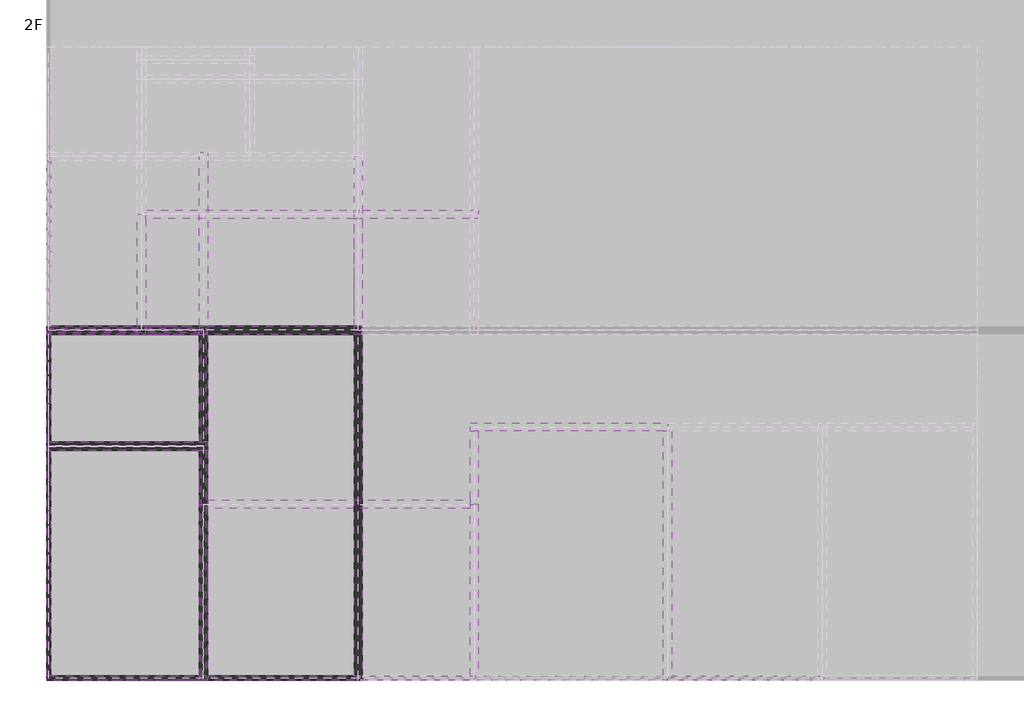
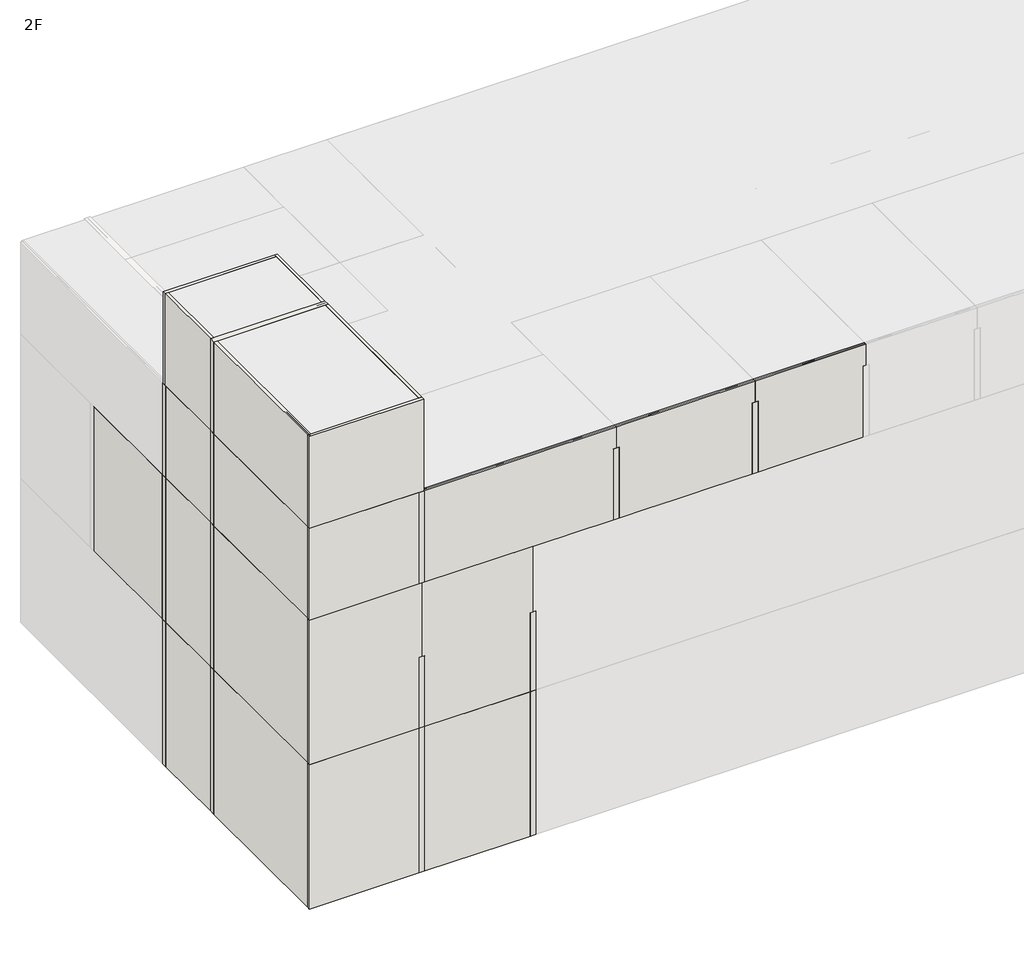
# One storey, part 1 of 3: 51 walls.
"""IFC4 building model written with IfcOpenShell, lengths in millimetres."""

from ifc_helpers import new_model, si_unit, frame, origin, place, context, project, spatial, polyline, outline, extrude, faceted_brep, element, save

model = new_model("IFC4")

# Units and contexts
model_context = context("Model", 3, world=origin())
ifc_project = project(units=[si_unit("LENGTHUNIT", "METRE", prefix="MILLI")], contexts=[model_context])

# Site, building, storey
site = spatial("IfcSite", under=ifc_project)
building = spatial("IfcBuilding", under=site)
storey = spatial("IfcBuildingStorey", under=building, Name="2F", Elevation=3500.0)

# Walls
placement = place(None, origin())
element("IfcWall", 1, ObjectType="WA211_Exterior-Cement Brick-90mm", at=placement, inside=storey, context=model_context, shape_type="SweptSolid", body=[
    extrude(outline(polyline([(49566.6521483, 163980.8614395), (53352.6521483, 163980.8614395), (53352.6521483, 163866.8614395), (49566.6521483, 163866.8614395), (49566.6521483, 163980.8614395)])), frame((0.0, 0.0, 3500.0), z_axis=(0.0, 0.0, 1.0), x_axis=(1.0, 0.0, 0.0)), (0.0, 0.0, 1.0), 5500.0),
])
element("IfcWall", 2, ObjectType="WA211_Exterior-Cement Brick-90mm", at=placement, inside=storey, context=model_context, shape_type="SweptSolid", body=[
    extrude(outline(polyline([(45516.6521483, 172816.8614395), (45516.6521483, 170030.8614395), (45402.6521483, 170030.8614395), (45402.6521483, 172816.8614395), (45516.6521483, 172816.8614395)])), frame((0.0, 0.0, 3500.0), z_axis=(0.0, 0.0, 1.0), x_axis=(1.0, 0.0, 0.0)), (0.0, 0.0, 1.0), 5500.0),
])
element("IfcWall", 3, ObjectType="WA211_Exterior-Cement Brick-90mm", at=placement, inside=storey, context=model_context, shape_type="SweptSolid", body=[
    extrude(outline(polyline([(45516.6521483, 169816.8614395), (45516.6521483, 163980.8614395), (45402.6521483, 163980.8614395), (45402.6521483, 169816.8614395), (45516.6521483, 169816.8614395)])), frame((0.0, 0.0, 3500.0), z_axis=(0.0, 0.0, 1.0), x_axis=(1.0, 0.0, 0.0)), (0.0, 0.0, 1.0), 5500.0),
])
element("IfcWall", 4, ObjectType="WA211_Exterior-Cement Brick-90mm", at=placement, inside=storey, context=model_context, shape_type="Brep", body=[
    faceted_brep([(49352.6521483, 163980.8614395, 3500.0), (45516.6521483, 163980.8614395, 3500.0), (45402.6521483, 163980.8614395, 3500.0), (45402.6521483, 163980.8614395, 9000.0), (45516.6521483, 163980.8614395, 9000.0), (49352.6521483, 163980.8614395, 9000.0), (49352.6521483, 163866.8614395, 3500.0), (49352.6521483, 163866.8614395, 9000.0), (45402.6521483, 163866.8614395, 9000.0), (45402.6521483, 163866.8614395, 3500.0)], [[[0, 1, 2, 3, 4, 5]], [[6, 7, 8, 9]], [[2, 1, 0, 6, 9]], [[5, 4, 3, 8, 7]], [[0, 5, 7, 6]], [[3, 2, 9, 8]]]),
])
element("IfcWall", 5, ObjectType="WA211_Exterior-Cement Brick-90mm", at=placement, inside=storey, context=model_context, shape_type="SweptSolid", body=[
    extrude(outline(polyline([(45516.6521483, 177316.8614395), (45516.6521483, 173030.8614395), (45402.6521483, 173030.8614395), (45402.6521483, 177316.8614395), (45516.6521483, 177316.8614395)])), frame((0.0, 0.0, 9000.0), z_axis=(0.0, 0.0, 1.0), x_axis=(1.0, 0.0, 0.0)), (0.0, 0.0, 1.0), 5500.0),
])
element("IfcWall", 6, ObjectType="WA211_Exterior-Cement Brick-90mm", at=placement, inside=storey, context=model_context, shape_type="SweptSolid", body=[
    extrude(outline(polyline([(45516.6521483, 172816.8614395), (45516.6521483, 170030.8614395), (45402.6521483, 170030.8614395), (45402.6521483, 172816.8614395), (45516.6521483, 172816.8614395)])), frame((0.0, 0.0, 9000.0), z_axis=(0.0, 0.0, 1.0), x_axis=(1.0, 0.0, 0.0)), (0.0, 0.0, 1.0), 5500.0),
])
element("IfcWall", 7, ObjectType="WA211_Exterior-Cement Brick-90mm", at=placement, inside=storey, context=model_context, shape_type="SweptSolid", body=[
    extrude(outline(polyline([(45516.6521483, 169816.8614395), (45516.6521483, 163980.8614395), (45402.6521483, 163980.8614395), (45402.6521483, 169816.8614395), (45516.6521483, 169816.8614395)])), frame((0.0, 0.0, 9000.0), z_axis=(0.0, 0.0, 1.0), x_axis=(1.0, 0.0, 0.0)), (0.0, 0.0, 1.0), 5500.0),
])
element("IfcWall", 8, ObjectType="WA211_Exterior-Cement Brick-90mm", at=placement, inside=storey, context=model_context, shape_type="Brep", body=[
    faceted_brep([(49352.6521483, 163980.8614395, 9000.0), (45516.6521483, 163980.8614395, 9000.0), (45402.6521483, 163980.8614395, 9000.0), (45402.6521483, 163980.8614395, 14500.0), (45516.6521483, 163980.8614395, 14500.0), (49459.6521483, 163980.8614395, 14500.0), (49459.6521483, 163980.8614395, 11700.0), (49352.6521483, 163980.8614395, 11700.0), (49352.6521483, 163866.8614395, 9000.0), (49352.6521483, 163866.8614395, 11700.0), (49459.6521483, 163866.8614395, 11700.0), (49459.6521483, 163866.8614395, 14500.0), (45402.6521483, 163866.8614395, 14500.0), (45402.6521483, 163866.8614395, 9000.0)], [[[0, 1, 2, 3, 4, 5, 6, 7]], [[8, 9, 10, 11, 12, 13]], [[2, 1, 0, 8, 13]], [[5, 4, 3, 12, 11]], [[3, 2, 13, 12]], [[6, 5, 11, 10]], [[6, 10, 9, 7]], [[0, 7, 9, 8]]]),
])
element("IfcWall", 9, ObjectType="WA211_Exterior-Cement Brick-90mm", at=placement, inside=storey, context=model_context, shape_type="SweptSolid", body=[
    extrude(outline(polyline([(9000.0, 53352.6521483), (12000.0, 53352.6521483), (12000.0, 53459.6521483), (14500.0, 53459.6521483), (14500.0, 49459.6521483), (11700.0, 49459.6521483), (11700.0, 49566.6521483), (9000.0, 49566.6521483), (9000.0, 53352.6521483)])), frame((0.0, 163866.8614395, 0.0), z_axis=(0.0, 1.0, 0.0), x_axis=(0.0, 0.0, 1.0)), (0.0, 0.0, 1.0), 114.0),
])
element("IfcWall", 10, ObjectType="WA211_Exterior-Cement Brick-90mm", at=placement, inside=storey, context=model_context, shape_type="SweptSolid", body=[
    extrude(outline(polyline([(14500.0, 65352.6521483), (17200.0, 65352.6521483), (17200.0, 65459.6521483), (18000.0, 65459.6521483), (18000.0, 61459.6521483), (17200.0, 61459.6521483), (17200.0, 61566.6521483), (14500.0, 61566.6521483), (14500.0, 65352.6521483)])), frame((0.0, 163866.8614395, 0.0), z_axis=(0.0, 1.0, 0.0), x_axis=(0.0, 0.0, 1.0)), (0.0, 0.0, 1.0), 114.0),
])
element("IfcWall", 11, ObjectType="WA211_Exterior-Cement Brick-90mm", at=placement, inside=storey, context=model_context, shape_type="SweptSolid", body=[
    extrude(outline(polyline([(14500.0, 61352.6521483), (17200.0, 61352.6521483), (17200.0, 61459.6521483), (18000.0, 61459.6521483), (18000.0, 56459.6521483), (17200.0, 56459.6521483), (17200.0, 56566.6521483), (14500.0, 56566.6521483), (14500.0, 61352.6521483)])), frame((0.0, 163866.8614395, 0.0), z_axis=(0.0, 1.0, 0.0), x_axis=(0.0, 0.0, 1.0)), (0.0, 0.0, 1.0), 114.0),
])
element("IfcWall", 12, ObjectType="WA211_Exterior-Cement Brick-90mm", at=placement, inside=storey, context=model_context, shape_type="SweptSolid", body=[
    extrude(outline(polyline([(14500.0, 56352.6521483), (17200.0, 56352.6521483), (17200.0, 56459.6521483), (18000.0, 56459.6521483), (18000.0, 49566.6521483), (14500.0, 49566.6521483), (14500.0, 56352.6521483)])), frame((0.0, 163866.8614395, 0.0), z_axis=(0.0, 1.0, 0.0), x_axis=(0.0, 0.0, 1.0)), (0.0, 0.0, 1.0), 114.0),
])
element("IfcWall", 13, ObjectType="WA211_Exterior-Cement Brick-90mm", at=placement, inside=storey, context=model_context, shape_type="SweptSolid", body=[
    extrude(outline(polyline([(45516.6521483, 172816.8614395), (45516.6521483, 170030.8614395), (45402.6521483, 170030.8614395), (45402.6521483, 172816.8614395), (45516.6521483, 172816.8614395)])), frame((0.0, 0.0, 14500.0), z_axis=(0.0, 0.0, 1.0), x_axis=(1.0, 0.0, 0.0)), (0.0, 0.0, 1.0), 3500.0),
])
element("IfcWall", 14, ObjectType="WA211_Exterior-Cement Brick-90mm", at=placement, inside=storey, context=model_context, shape_type="SweptSolid", body=[
    extrude(outline(polyline([(45516.6521483, 169816.8614395), (45516.6521483, 163980.8614395), (45402.6521483, 163980.8614395), (45402.6521483, 169816.8614395), (45516.6521483, 169816.8614395)])), frame((0.0, 0.0, 14500.0), z_axis=(0.0, 0.0, 1.0), x_axis=(1.0, 0.0, 0.0)), (0.0, 0.0, 1.0), 3500.0),
])
element("IfcWall", 15, ObjectType="WA211_Exterior-Cement Brick-90mm", at=placement, inside=storey, context=model_context, shape_type="Brep", body=[
    faceted_brep([(49352.6521483, 163980.8614395, 14500.0), (45516.6521483, 163980.8614395, 14500.0), (45402.6521483, 163980.8614395, 14500.0), (45402.6521483, 163980.8614395, 18000.0), (45516.6521483, 163980.8614395, 18000.0), (49352.6521483, 163980.8614395, 18000.0), (49352.6521483, 163866.8614395, 14500.0), (49352.6521483, 163866.8614395, 18000.0), (45402.6521483, 163866.8614395, 18000.0), (45402.6521483, 163866.8614395, 14500.0)], [[[0, 1, 2, 3, 4, 5]], [[6, 7, 8, 9]], [[2, 1, 0, 6, 9]], [[5, 4, 3, 8, 7]], [[0, 5, 7, 6]], [[3, 2, 9, 8]]]),
])
element("IfcWall", 16, ObjectType="WA211_Exterior-Cement Brick-90mm", at=placement, inside=storey, context=model_context, shape_type="Brep", body=[
    faceted_brep([(49402.6521483, 172980.8614395, 18000.0), (49402.6521483, 172866.8614395, 18000.0), (49402.6521483, 170030.8614395, 18000.0), (49402.6521483, 170030.8614395, 21500.0), (49402.6521483, 172866.8614395, 21500.0), (49402.6521483, 172980.8614395, 21500.0), (49516.6521483, 172980.8614395, 18000.0), (49516.6521483, 172980.8614395, 21500.0), (49516.6521483, 170030.8614395, 21500.0), (49516.6521483, 170030.8614395, 18000.0)], [[[0, 1, 2, 3, 4, 5]], [[6, 7, 8, 9]], [[2, 1, 0, 6, 9]], [[5, 4, 3, 8, 7]], [[0, 5, 7, 6]], [[3, 2, 9, 8]]]),
])
element("IfcWall", 17, ObjectType="WA211_Exterior-Cement Brick-90mm", at=placement, inside=storey, context=model_context, shape_type="SweptSolid", body=[
    extrude(outline(polyline([(45516.6521483, 172866.8614395), (45516.6521483, 170030.8614395), (45402.6521483, 170030.8614395), (45402.6521483, 172866.8614395), (45516.6521483, 172866.8614395)])), frame((0.0, 0.0, 18000.0), z_axis=(0.0, 0.0, 1.0), x_axis=(1.0, 0.0, 0.0)), (0.0, 0.0, 1.0), 3500.0),
])
element("IfcWall", 18, ObjectType="WA211_Exterior-Cement Brick-90mm", at=placement, inside=storey, context=model_context, shape_type="Brep", body=[
    faceted_brep([(45402.6521483, 172866.8614395, 18000.0), (45516.6521483, 172866.8614395, 18000.0), (49402.6521483, 172866.8614395, 18000.0), (49402.6521483, 172866.8614395, 21500.0), (45516.6521483, 172866.8614395, 21500.0), (45402.6521483, 172866.8614395, 21500.0), (45402.6521483, 172980.8614395, 18000.0), (45402.6521483, 172980.8614395, 21500.0), (49402.6521483, 172980.8614395, 21500.0), (49402.6521483, 172980.8614395, 18000.0)], [[[0, 1, 2, 3, 4, 5]], [[6, 7, 8, 9]], [[2, 1, 0, 6, 9]], [[5, 4, 3, 8, 7]], [[0, 5, 7, 6]], [[3, 2, 9, 8]]]),
])
element("IfcWall", 19, ObjectType="WA211_Exterior-Cement Brick-90mm", at=placement, inside=storey, context=model_context, shape_type="SweptSolid", body=[
    extrude(outline(polyline([(45516.6521483, 169816.8614395), (45516.6521483, 163980.8614395), (45402.6521483, 163980.8614395), (45402.6521483, 169816.8614395), (45516.6521483, 169816.8614395)])), frame((0.0, 0.0, 18000.0), z_axis=(0.0, 0.0, 1.0), x_axis=(1.0, 0.0, 0.0)), (0.0, 0.0, 1.0), 3500.0),
])
element("IfcWall", 20, ObjectType="WA211_Exterior-Cement Brick-90mm", at=placement, inside=storey, context=model_context, shape_type="Brep", body=[
    faceted_brep([(49516.6521483, 163980.8614395, 18000.0), (49402.6521483, 163980.8614395, 18000.0), (45516.6521483, 163980.8614395, 18000.0), (45402.6521483, 163980.8614395, 18000.0), (45402.6521483, 163980.8614395, 21500.0), (45516.6521483, 163980.8614395, 21500.0), (49402.6521483, 163980.8614395, 21500.0), (49516.6521483, 163980.8614395, 21500.0), (49516.6521483, 163866.8614395, 18000.0), (49516.6521483, 163866.8614395, 21500.0), (45402.6521483, 163866.8614395, 21500.0), (45402.6521483, 163866.8614395, 18000.0)], [[[0, 1, 2, 3, 4, 5, 6, 7]], [[8, 9, 10, 11]], [[3, 2, 1, 0, 8, 11]], [[7, 6, 5, 4, 10, 9]], [[0, 7, 9, 8]], [[4, 3, 11, 10]]]),
])
element("IfcWall", 21, ObjectType="WA211_Exterior-Cement Brick-90mm", at=placement, inside=storey, context=model_context, shape_type="SweptSolid", body=[
    extrude(outline(polyline([(49402.6521483, 163980.8614395), (49402.6521483, 169816.8614395), (49516.6521483, 169816.8614395), (49516.6521483, 163980.8614395), (49402.6521483, 163980.8614395)])), frame((0.0, 0.0, 18000.0), z_axis=(0.0, 0.0, 1.0), x_axis=(1.0, 0.0, 0.0)), (0.0, 0.0, 1.0), 3500.0),
])
element("IfcWall", 22, ObjectType="WA221_Interior-Cement Block-190mm", at=placement, inside=storey, context=model_context, shape_type="SweptSolid", body=[
    extrude(outline(polyline([(49566.6521483, 173030.8614395), (53352.6521483, 173030.8614395), (53352.6521483, 172816.8614395), (49566.6521483, 172816.8614395), (49566.6521483, 173030.8614395)])), frame((0.0, 0.0, 3500.0), z_axis=(0.0, 0.0, 1.0), x_axis=(1.0, 0.0, 0.0)), (0.0, 0.0, 1.0), 5500.0),
])
element("IfcWall", 23, ObjectType="WA221_Interior-Cement Block-190mm", at=placement, inside=storey, context=model_context, shape_type="Brep", body=[
    faceted_brep([(45402.6521483, 172816.8614395, 3500.0), (45516.6521483, 172816.8614395, 3500.0), (49352.6521483, 172816.8614395, 3500.0), (49352.6521483, 172816.8614395, 9000.0), (45516.6521483, 172816.8614395, 9000.0), (45402.6521483, 172816.8614395, 9000.0), (45402.6521483, 173030.8614395, 3500.0), (45402.6521483, 173030.8614395, 9000.0), (45516.6521483, 173030.8614395, 9000.0), (49352.6521483, 173030.8614395, 9000.0), (49352.6521483, 173030.8614395, 3500.0), (45516.6521483, 173030.8614395, 3500.0)], [[[0, 1, 2, 3, 4, 5]], [[6, 7, 8, 9, 10, 11]], [[2, 1, 0, 6, 11, 10]], [[5, 4, 3, 9, 8, 7]], [[0, 5, 7, 6]], [[3, 2, 10, 9]]]),
])
element("IfcWall", 24, ObjectType="WA221_Interior-Cement Block-190mm", at=placement, inside=storey, context=model_context, shape_type="Brep", body=[
    faceted_brep([(53566.6521483, 163866.8614395, 3500.0), (53566.6521483, 163980.8614395, 3500.0), (53566.6521483, 172816.8614395, 3500.0), (53566.6521483, 173030.8614395, 3500.0), (53566.6521483, 173030.8614395, 9000.0), (53566.6521483, 172816.8614395, 9000.0), (53566.6521483, 163980.8614395, 9000.0), (53566.6521483, 163866.8614395, 9000.0), (53352.6521483, 163866.8614395, 3500.0), (53352.6521483, 163866.8614395, 9000.0), (53352.6521483, 163980.8614395, 9000.0), (53352.6521483, 172816.8614395, 9000.0), (53352.6521483, 173030.8614395, 9000.0), (53352.6521483, 173030.8614395, 3500.0), (53352.6521483, 172816.8614395, 3500.0), (53352.6521483, 163980.8614395, 3500.0)], [[[0, 1, 2, 3, 4, 5, 6, 7]], [[8, 9, 10, 11, 12, 13, 14, 15]], [[3, 2, 1, 0, 8, 15, 14, 13]], [[7, 6, 5, 4, 12, 11, 10, 9]], [[0, 7, 9, 8]], [[4, 3, 13, 12]]]),
])
element("IfcWall", 25, ObjectType="WA221_Interior-Cement Block-190mm", at=placement, inside=storey, context=model_context, shape_type="Brep", body=[
    faceted_brep([(49352.6521483, 173030.8614395, 3500.0), (49352.6521483, 172816.8614395, 3500.0), (49352.6521483, 170030.8614395, 3500.0), (49352.6521483, 170030.8614395, 9000.0), (49352.6521483, 172816.8614395, 9000.0), (49352.6521483, 173030.8614395, 9000.0), (49566.6521483, 173030.8614395, 3500.0), (49566.6521483, 173030.8614395, 9000.0), (49566.6521483, 172816.8614395, 9000.0), (49566.6521483, 170030.8614395, 9000.0), (49566.6521483, 170030.8614395, 3500.0), (49566.6521483, 172816.8614395, 3500.0)], [[[0, 1, 2, 3, 4, 5]], [[6, 7, 8, 9, 10, 11]], [[2, 1, 0, 6, 11, 10]], [[5, 4, 3, 9, 8, 7]], [[0, 5, 7, 6]], [[3, 2, 10, 9]]]),
])
element("IfcWall", 26, ObjectType="WA221_Interior-Cement Block-190mm", at=placement, inside=storey, context=model_context, shape_type="Brep", body=[
    faceted_brep([(49352.6521483, 169816.8614395, 3500.0), (49352.6521483, 163980.8614395, 3500.0), (49352.6521483, 163866.8614395, 3500.0), (49352.6521483, 163866.8614395, 9000.0), (49352.6521483, 163980.8614395, 9000.0), (49352.6521483, 169816.8614395, 9000.0), (49566.6521483, 169816.8614395, 3500.0), (49566.6521483, 169816.8614395, 9000.0), (49566.6521483, 163980.8614395, 9000.0), (49566.6521483, 163866.8614395, 9000.0), (49566.6521483, 163866.8614395, 3500.0), (49566.6521483, 163980.8614395, 3500.0)], [[[0, 1, 2, 3, 4, 5]], [[6, 7, 8, 9, 10, 11]], [[2, 1, 0, 6, 11, 10]], [[5, 4, 3, 9, 8, 7]], [[3, 2, 10, 9]], [[0, 5, 7, 6]]]),
])
element("IfcWall", 27, ObjectType="WA221_Interior-Cement Block-190mm", at=placement, inside=storey, context=model_context, shape_type="Brep", body=[
    faceted_brep([(45402.6521483, 169816.8614395, 3500.0), (45516.6521483, 169816.8614395, 3500.0), (49352.6521483, 169816.8614395, 3500.0), (49566.6521483, 169816.8614395, 3500.0), (49566.6521483, 169816.8614395, 9000.0), (49352.6521483, 169816.8614395, 9000.0), (45516.6521483, 169816.8614395, 9000.0), (45402.6521483, 169816.8614395, 9000.0), (45402.6521483, 170030.8614395, 3500.0), (45402.6521483, 170030.8614395, 9000.0), (45516.6521483, 170030.8614395, 9000.0), (49352.6521483, 170030.8614395, 9000.0), (49566.6521483, 170030.8614395, 9000.0), (49566.6521483, 170030.8614395, 3500.0), (49352.6521483, 170030.8614395, 3500.0), (45516.6521483, 170030.8614395, 3500.0)], [[[0, 1, 2, 3, 4, 5, 6, 7]], [[8, 9, 10, 11, 12, 13, 14, 15]], [[3, 2, 1, 0, 8, 15, 14, 13]], [[7, 6, 5, 4, 12, 11, 10, 9]], [[0, 7, 9, 8]], [[4, 3, 13, 12]]]),
])
element("IfcWall", 28, ObjectType="WA221_Interior-Cement Block-190mm", at=placement, inside=storey, context=model_context, shape_type="Brep", body=[
    faceted_brep([(53566.6521483, 172923.8614395, 9000.0), (53566.6521483, 173030.8614395, 9000.0), (53566.6521483, 177316.8614395, 9000.0), (53566.6521483, 177316.8614395, 11700.0), (53566.6521483, 177423.8614395, 11700.0), (53566.6521483, 177423.8614395, 12400.0), (53566.6521483, 173030.8614395, 12400.0), (53566.6521483, 172816.8614395, 12400.0), (53566.6521483, 172816.8614395, 12000.0), (53566.6521483, 172923.8614395, 12000.0), (53352.6521483, 172923.8614395, 9000.0), (53352.6521483, 172923.8614395, 12000.0), (53352.6521483, 172816.8614395, 12000.0), (53352.6521483, 172816.8614395, 12400.0), (53352.6521483, 177423.8614395, 12400.0), (53352.6521483, 177423.8614395, 11700.0), (53352.6521483, 177316.8614395, 11700.0), (53352.6521483, 177316.8614395, 9000.0)], [[[0, 1, 2, 3, 4, 5, 6, 7, 8, 9]], [[10, 11, 12, 13, 14, 15, 16, 17]], [[2, 1, 0, 10, 17]], [[7, 6, 5, 14, 13]], [[0, 9, 11, 10]], [[8, 12, 11, 9]], [[8, 7, 13, 12]], [[5, 4, 15, 14]], [[15, 4, 3, 16]], [[3, 2, 17, 16]]]),
])
element("IfcWall", 29, ObjectType="WA221_Interior-Cement Block-190mm", at=placement, inside=storey, context=model_context, shape_type="Brep", body=[
    faceted_brep([(53566.6521483, 163866.8614395, 9000.0), (53566.6521483, 163980.8614395, 9000.0), (53566.6521483, 172816.8614395, 9000.0), (53566.6521483, 172923.8614395, 9000.0), (53566.6521483, 172923.8614395, 12000.0), (53566.6521483, 172816.8614395, 12000.0), (53566.6521483, 163980.8614395, 12000.0), (53566.6521483, 163866.8614395, 12000.0), (53352.6521483, 163866.8614395, 9000.0), (53352.6521483, 163866.8614395, 12000.0), (53352.6521483, 163980.8614395, 12000.0), (53352.6521483, 172816.8614395, 12000.0), (53352.6521483, 172923.8614395, 12000.0), (53352.6521483, 172923.8614395, 9000.0), (53352.6521483, 163980.8614395, 9000.0), (53459.6521483, 163866.8614395, 12000.0)], [[[0, 1, 2, 3, 4, 5, 6, 7]], [[8, 9, 10, 11, 12, 13, 14]], [[3, 2, 1, 0, 8, 14, 13]], [[4, 3, 13, 12]], [[7, 6, 5, 4, 12, 11, 10, 9, 15]], [[0, 7, 15, 9, 8]]]),
])
element("IfcWall", 30, ObjectType="WA221_Interior-Cement Block-190mm", at=placement, inside=storey, context=model_context, shape_type="Brep", body=[
    faceted_brep([(45402.6521483, 172816.8614395, 9000.0), (45516.6521483, 172816.8614395, 9000.0), (49352.6521483, 172816.8614395, 9000.0), (49566.6521483, 172816.8614395, 9000.0), (49566.6521483, 172816.8614395, 14500.0), (49352.6521483, 172816.8614395, 14500.0), (45516.6521483, 172816.8614395, 14500.0), (45402.6521483, 172816.8614395, 14500.0), (45402.6521483, 173030.8614395, 9000.0), (45402.6521483, 173030.8614395, 14500.0), (45516.6521483, 173030.8614395, 14500.0), (49566.6521483, 173030.8614395, 14500.0), (49566.6521483, 173030.8614395, 11700.0), (49566.6521483, 173030.8614395, 9000.0), (49352.6521483, 173030.8614395, 9000.0), (45516.6521483, 173030.8614395, 9000.0)], [[[0, 1, 2, 3, 4, 5, 6, 7]], [[8, 9, 10, 11, 12, 13, 14, 15]], [[3, 2, 1, 0, 8, 15, 14, 13]], [[7, 6, 5, 4, 11, 10, 9]], [[0, 7, 9, 8]], [[3, 13, 12, 11, 4]]]),
])
element("IfcWall", 31, ObjectType="WA221_Interior-Cement Block-190mm", at=placement, inside=storey, context=model_context, shape_type="Brep", body=[
    faceted_brep([(49352.6521483, 177530.8614395, 9000.0), (49352.6521483, 177316.8614395, 9000.0), (49352.6521483, 173030.8614395, 9000.0), (49352.6521483, 173030.8614395, 11700.0), (49352.6521483, 177316.8614395, 11700.0), (49352.6521483, 177530.8614395, 11700.0), (49566.6521483, 177530.8614395, 9000.0), (49566.6521483, 177530.8614395, 11700.0), (49566.6521483, 177316.8614395, 11700.0), (49566.6521483, 173030.8614395, 11700.0), (49566.6521483, 173030.8614395, 9000.0), (49566.6521483, 177316.8614395, 9000.0)], [[[0, 1, 2, 3, 4, 5]], [[6, 7, 8, 9, 10, 11]], [[2, 1, 0, 6, 11, 10]], [[5, 4, 3, 9, 8, 7]], [[0, 5, 7, 6]], [[3, 2, 10, 9]]]),
])
element("IfcWall", 32, ObjectType="WA221_Interior-Cement Block-190mm", at=placement, inside=storey, context=model_context, shape_type="Brep", body=[
    faceted_brep([(49566.6521483, 170030.8614395, 14500.0), (49566.6521483, 170030.8614395, 9000.0), (49352.6521483, 170030.8614395, 9000.0), (45516.6521483, 170030.8614395, 9000.0), (45402.6521483, 170030.8614395, 9000.0), (45402.6521483, 170030.8614395, 14500.0), (45516.6521483, 170030.8614395, 14500.0), (49352.6521483, 170030.8614395, 14500.0), (49566.6521483, 169816.8614395, 9000.0), (49566.6521483, 169816.8614395, 11700.0), (49566.6521483, 169816.8614395, 14500.0), (45516.6521483, 169816.8614395, 14500.0), (45402.6521483, 169816.8614395, 14500.0), (45402.6521483, 169816.8614395, 9000.0), (45516.6521483, 169816.8614395, 9000.0), (49352.6521483, 169816.8614395, 9000.0)], [[[0, 1, 2, 3, 4, 5, 6, 7]], [[8, 9, 10, 11, 12, 13, 14, 15]], [[4, 3, 2, 1, 8, 15, 14, 13]], [[0, 7, 6, 5, 12, 11, 10]], [[5, 4, 13, 12]], [[0, 10, 9, 8, 1]]]),
])
element("IfcWall", 33, ObjectType="WA221_Interior-Cement Block-190mm", at=placement, inside=storey, context=model_context, shape_type="SweptSolid", body=[
    extrude(outline(polyline([(49352.6521483, 170030.8614395), (49352.6521483, 172816.8614395), (49566.6521483, 172816.8614395), (49566.6521483, 170030.8614395), (49352.6521483, 170030.8614395)])), frame((0.0, 0.0, 9000.0), z_axis=(0.0, 0.0, 1.0), x_axis=(1.0, 0.0, 0.0)), (0.0, 0.0, 1.0), 5500.0),
])
element("IfcWall", 34, ObjectType="WA221_Interior-Cement Block-190mm", at=placement, inside=storey, context=model_context, shape_type="Brep", body=[
    faceted_brep([(49352.6521483, 169816.8614395, 9000.0), (49352.6521483, 163980.8614395, 9000.0), (49352.6521483, 163866.8614395, 9000.0), (49352.6521483, 163866.8614395, 11700.0), (49352.6521483, 163980.8614395, 11700.0), (49352.6521483, 169816.8614395, 11700.0), (49566.6521483, 169816.8614395, 9000.0), (49566.6521483, 169816.8614395, 11700.0), (49566.6521483, 163980.8614395, 11700.0), (49566.6521483, 163866.8614395, 11700.0), (49566.6521483, 163866.8614395, 9000.0), (49566.6521483, 163980.8614395, 9000.0), (49459.6521483, 163866.8614395, 11700.0)], [[[0, 1, 2, 3, 4, 5]], [[6, 7, 8, 9, 10, 11]], [[2, 1, 0, 6, 11, 10]], [[5, 4, 3, 12, 9, 8, 7]], [[0, 5, 7, 6]], [[3, 2, 10, 9, 12]]]),
])
element("IfcWall", 35, ObjectType="WA221_Interior-Cement Block-190mm", at=placement, inside=storey, context=model_context, shape_type="Brep", body=[
    faceted_brep([(61352.6521483, 170316.8614395, 14500.0), (61352.6521483, 163980.8614395, 14500.0), (61352.6521483, 163866.8614395, 14500.0), (61352.6521483, 163866.8614395, 17200.0), (61352.6521483, 163980.8614395, 17200.0), (61352.6521483, 170316.8614395, 17200.0), (61566.6521483, 170316.8614395, 14500.0), (61566.6521483, 170316.8614395, 17200.0), (61566.6521483, 163980.8614395, 17200.0), (61566.6521483, 163866.8614395, 17200.0), (61566.6521483, 163866.8614395, 14500.0), (61566.6521483, 163980.8614395, 14500.0), (61459.6521483, 170316.8614395, 14500.0), (61459.6521483, 163866.8614395, 17200.0), (61459.6521483, 170316.8614395, 17200.0)], [[[0, 1, 2, 3, 4, 5]], [[6, 7, 8, 9, 10, 11]], [[2, 1, 0, 12, 6, 11, 10]], [[5, 4, 3, 13, 9, 8, 7, 14]], [[3, 2, 10, 9, 13]], [[0, 5, 14, 7, 6, 12]]]),
])
element("IfcWall", 36, ObjectType="WA221_Interior-Cement Block-190mm", at=placement, inside=storey, context=model_context, shape_type="Brep", body=[
    faceted_brep([(56566.6521483, 163866.8614395, 14500.0), (56566.6521483, 163980.8614395, 14500.0), (56566.6521483, 168423.8614395, 14500.0), (56566.6521483, 168423.8614395, 17200.0), (56566.6521483, 163980.8614395, 17200.0), (56566.6521483, 163866.8614395, 17200.0), (56352.6521483, 163866.8614395, 14500.0), (56352.6521483, 163866.8614395, 17200.0), (56352.6521483, 163980.8614395, 17200.0), (56352.6521483, 168316.8614395, 17200.0), (56352.6521483, 168423.8614395, 17200.0), (56352.6521483, 168423.8614395, 14500.0), (56352.6521483, 168316.8614395, 14500.0), (56352.6521483, 163980.8614395, 14500.0), (56459.6521483, 163866.8614395, 17200.0)], [[[0, 1, 2, 3, 4, 5]], [[6, 7, 8, 9, 10, 11, 12, 13]], [[2, 1, 0, 6, 13, 12, 11]], [[3, 2, 11, 10]], [[5, 4, 3, 10, 9, 8, 7, 14]], [[0, 5, 14, 7, 6]]]),
])
element("IfcWall", 37, ObjectType="WA221_Interior-Cement Block-190mm", at=placement, inside=storey, context=model_context, shape_type="Brep", body=[
    faceted_brep([(56352.6521483, 170316.8614395, 14500.0), (56566.6521483, 170316.8614395, 14500.0), (61352.6521483, 170316.8614395, 14500.0), (61459.6521483, 170316.8614395, 14500.0), (61459.6521483, 170316.8614395, 17200.0), (61352.6521483, 170316.8614395, 17200.0), (56566.6521483, 170316.8614395, 17200.0), (56352.6521483, 170316.8614395, 17200.0), (56352.6521483, 170530.8614395, 14500.0), (56352.6521483, 170530.8614395, 17200.0), (61459.6521483, 170530.8614395, 17200.0), (61459.6521483, 170530.8614395, 14500.0)], [[[0, 1, 2, 3, 4, 5, 6, 7]], [[8, 9, 10, 11]], [[3, 2, 1, 0, 8, 11]], [[4, 3, 11, 10]], [[7, 6, 5, 4, 10, 9]], [[0, 7, 9, 8]]]),
])
element("IfcWall", 38, ObjectType="WA221_Interior-Cement Block-190mm", at=placement, inside=storey, context=model_context, shape_type="Brep", body=[
    faceted_brep([(56566.6521483, 168423.8614395, 14500.0), (56566.6521483, 170316.8614395, 14500.0), (56566.6521483, 170316.8614395, 17200.0), (56566.6521483, 168423.8614395, 17200.0), (56352.6521483, 168423.8614395, 14500.0), (56352.6521483, 168423.8614395, 17200.0), (56352.6521483, 168530.8614395, 17200.0), (56352.6521483, 170316.8614395, 17200.0), (56352.6521483, 170316.8614395, 14500.0), (56352.6521483, 168530.8614395, 14500.0)], [[[0, 1, 2, 3]], [[4, 5, 6, 7, 8, 9]], [[1, 0, 4, 9, 8]], [[3, 2, 7, 6, 5]], [[0, 3, 5, 4]], [[2, 1, 8, 7]]]),
])
element("IfcWall", 39, ObjectType="WA221_Interior-Cement Block-190mm", at=placement, inside=storey, context=model_context, shape_type="Brep", body=[
    faceted_brep([(49352.6521483, 168423.8614395, 18000.0), (49352.6521483, 168423.8614395, 14500.0), (49352.6521483, 163980.8614395, 14500.0), (49352.6521483, 163866.8614395, 14500.0), (49352.6521483, 163866.8614395, 18000.0), (49352.6521483, 163980.8614395, 18000.0), (49566.6521483, 168423.8614395, 14500.0), (49566.6521483, 168423.8614395, 18000.0), (49566.6521483, 163980.8614395, 18000.0), (49566.6521483, 163866.8614395, 18000.0), (49566.6521483, 163866.8614395, 14500.0), (49566.6521483, 163980.8614395, 14500.0), (49566.6521483, 168316.8614395, 14500.0)], [[[0, 1, 2, 3, 4, 5]], [[6, 7, 8, 9, 10, 11, 12]], [[3, 2, 1, 6, 12, 11, 10]], [[0, 5, 4, 9, 8, 7]], [[0, 7, 6, 1]], [[4, 3, 10, 9]]]),
])
element("IfcWall", 40, ObjectType="WA221_Interior-Cement Block-190mm", at=placement, inside=storey, context=model_context, shape_type="Brep", body=[
    faceted_brep([(56352.6521483, 168530.8614395, 14500.0), (49566.6521483, 168530.8614395, 14500.0), (49566.6521483, 168530.8614395, 17200.0), (56352.6521483, 168530.8614395, 17200.0), (56352.6521483, 168316.8614395, 14500.0), (56352.6521483, 168316.8614395, 17200.0), (49566.6521483, 168316.8614395, 17200.0), (49566.6521483, 168316.8614395, 14500.0), (56352.6521483, 168423.8614395, 14500.0), (49566.6521483, 168423.8614395, 14500.0), (56352.6521483, 168423.8614395, 17200.0)], [[[0, 1, 2, 3]], [[4, 5, 6, 7]], [[1, 0, 8, 4, 7, 9]], [[3, 2, 6, 5, 10]], [[0, 3, 10, 5, 4, 8]], [[2, 1, 9, 7, 6]]]),
])
element("IfcWall", 41, ObjectType="WA221_Interior-Cement Block-190mm", at=placement, inside=storey, context=model_context, shape_type="Brep", body=[
    faceted_brep([(47966.6521483, 175816.8614395, 14500.0), (53352.6521483, 175816.8614395, 14500.0), (53459.6521483, 175816.8614395, 14500.0), (53459.6521483, 175816.8614395, 17200.0), (53352.6521483, 175816.8614395, 17200.0), (47966.6521483, 175816.8614395, 17200.0), (47966.6521483, 176030.8614395, 14500.0), (47966.6521483, 176030.8614395, 17200.0), (53352.6521483, 176030.8614395, 17200.0), (53459.6521483, 176030.8614395, 17200.0), (53459.6521483, 176030.8614395, 14500.0), (53352.6521483, 176030.8614395, 14500.0), (47966.6521483, 175923.8614395, 14500.0)], [[[0, 1, 2, 3, 4, 5]], [[6, 7, 8, 9, 10, 11]], [[2, 1, 0, 12, 6, 11, 10]], [[3, 2, 10, 9]], [[5, 4, 3, 9, 8, 7]], [[0, 5, 7, 6, 12]]]),
])
element("IfcWall", 42, ObjectType="WA221_Interior-Cement Block-190mm", at=placement, inside=storey, context=model_context, shape_type="Brep", body=[
    faceted_brep([(53459.6521483, 175816.8614395, 14500.0), (53566.6521483, 175816.8614395, 14500.0), (56352.6521483, 175816.8614395, 14500.0), (56566.6521483, 175816.8614395, 14500.0), (56566.6521483, 175816.8614395, 17200.0), (56352.6521483, 175816.8614395, 17200.0), (53566.6521483, 175816.8614395, 17200.0), (53459.6521483, 175816.8614395, 17200.0), (53459.6521483, 176030.8614395, 14500.0), (53459.6521483, 176030.8614395, 17200.0), (53566.6521483, 176030.8614395, 17200.0), (56352.6521483, 176030.8614395, 17200.0), (56566.6521483, 176030.8614395, 17200.0), (56566.6521483, 176030.8614395, 14500.0), (56352.6521483, 176030.8614395, 14500.0), (53566.6521483, 176030.8614395, 14500.0)], [[[0, 1, 2, 3, 4, 5, 6, 7]], [[8, 9, 10, 11, 12, 13, 14, 15]], [[3, 2, 1, 0, 8, 15, 14, 13]], [[7, 6, 5, 4, 12, 11, 10, 9]], [[0, 7, 9, 8]], [[4, 3, 13, 12]]]),
])
element("IfcWall", 43, ObjectType="WA221_Interior-Cement Block-190mm", at=placement, inside=storey, context=model_context, shape_type="Brep", body=[
    faceted_brep([(47752.6521483, 175923.8614395, 18000.0), (47752.6521483, 175923.8614395, 14500.0), (47752.6521483, 173030.8614395, 14500.0), (47752.6521483, 172816.8614395, 14500.0), (47752.6521483, 172816.8614395, 18000.0), (47752.6521483, 173030.8614395, 18000.0), (47966.6521483, 175923.8614395, 14500.0), (47966.6521483, 175923.8614395, 18000.0), (47966.6521483, 173030.8614395, 18000.0), (47966.6521483, 172816.8614395, 18000.0), (47966.6521483, 172816.8614395, 14500.0), (47966.6521483, 173030.8614395, 14500.0), (47966.6521483, 175816.8614395, 14500.0)], [[[0, 1, 2, 3, 4, 5]], [[6, 7, 8, 9, 10, 11, 12]], [[3, 2, 1, 6, 12, 11, 10]], [[0, 5, 4, 9, 8, 7]], [[0, 7, 6, 1]], [[4, 3, 10, 9]]]),
])
element("IfcWall", 44, ObjectType="WA221_Interior-Cement Block-190mm", at=placement, inside=storey, context=model_context, shape_type="SweptSolid", body=[
    extrude(outline(polyline([(49352.6521483, 172816.8614395), (47966.6521483, 172816.8614395), (47966.6521483, 173030.8614395), (49352.6521483, 173030.8614395), (49352.6521483, 172816.8614395)])), frame((0.0, 0.0, 14500.0), z_axis=(0.0, 0.0, 1.0), x_axis=(1.0, 0.0, 0.0)), (0.0, 0.0, 1.0), 3500.0),
])
element("IfcWall", 45, ObjectType="WA221_Interior-Cement Block-190mm", at=placement, inside=storey, context=model_context, shape_type="Brep", body=[
    faceted_brep([(53566.6521483, 173030.8614395, 14500.0), (53352.6521483, 173030.8614395, 14500.0), (49566.6521483, 173030.8614395, 14500.0), (49566.6521483, 173030.8614395, 17200.0), (53352.6521483, 173030.8614395, 17200.0), (53566.6521483, 173030.8614395, 17200.0), (53566.6521483, 172816.8614395, 14500.0), (53566.6521483, 172816.8614395, 17200.0), (49566.6521483, 172816.8614395, 17200.0), (49566.6521483, 172816.8614395, 14500.0)], [[[0, 1, 2, 3, 4, 5]], [[6, 7, 8, 9]], [[2, 1, 0, 6, 9]], [[5, 4, 3, 8, 7]], [[0, 5, 7, 6]], [[3, 2, 9, 8]]]),
])
element("IfcWall", 46, ObjectType="WA221_Interior-Cement Block-190mm", at=placement, inside=storey, context=model_context, shape_type="Brep", body=[
    faceted_brep([(53352.6521483, 175816.8614395, 14500.0), (53352.6521483, 173030.8614395, 14500.0), (53352.6521483, 173030.8614395, 17200.0), (53352.6521483, 175816.8614395, 17200.0), (53566.6521483, 175816.8614395, 14500.0), (53566.6521483, 175816.8614395, 17200.0), (53566.6521483, 173030.8614395, 17200.0), (53566.6521483, 173030.8614395, 14500.0), (53459.6521483, 175816.8614395, 14500.0), (53459.6521483, 175816.8614395, 17200.0)], [[[0, 1, 2, 3]], [[4, 5, 6, 7]], [[1, 0, 8, 4, 7]], [[3, 2, 6, 5, 9]], [[0, 3, 9, 5, 4, 8]], [[2, 1, 7, 6]]]),
])
element("IfcWall", 47, ObjectType="WA221_Interior-Cement Block-190mm", at=placement, inside=storey, context=model_context, shape_type="Brep", body=[
    faceted_brep([(47752.6521483, 173030.8614395, 14500.0), (45516.6521483, 173030.8614395, 14500.0), (45402.6521483, 173030.8614395, 14500.0), (45402.6521483, 173030.8614395, 18000.0), (45516.6521483, 173030.8614395, 18000.0), (47752.6521483, 173030.8614395, 18000.0), (47752.6521483, 172816.8614395, 14500.0), (47752.6521483, 172816.8614395, 18000.0), (45516.6521483, 172816.8614395, 18000.0), (45402.6521483, 172816.8614395, 18000.0), (45402.6521483, 172816.8614395, 14500.0), (45516.6521483, 172816.8614395, 14500.0)], [[[0, 1, 2, 3, 4, 5]], [[6, 7, 8, 9, 10, 11]], [[2, 1, 0, 6, 11, 10]], [[5, 4, 3, 9, 8, 7]], [[0, 5, 7, 6]], [[3, 2, 10, 9]]]),
])
element("IfcWall", 48, ObjectType="WA221_Interior-Cement Block-190mm", at=placement, inside=storey, context=model_context, shape_type="Brep", body=[
    faceted_brep([(45402.6521483, 169816.8614395, 14500.0), (45516.6521483, 169816.8614395, 14500.0), (49352.6521483, 169816.8614395, 14500.0), (49566.6521483, 169816.8614395, 14500.0), (49566.6521483, 169816.8614395, 18000.0), (49352.6521483, 169816.8614395, 18000.0), (45516.6521483, 169816.8614395, 18000.0), (45402.6521483, 169816.8614395, 18000.0), (45402.6521483, 170030.8614395, 14500.0), (45402.6521483, 170030.8614395, 18000.0), (45516.6521483, 170030.8614395, 18000.0), (49352.6521483, 170030.8614395, 18000.0), (49566.6521483, 170030.8614395, 18000.0), (49566.6521483, 170030.8614395, 14500.0), (49352.6521483, 170030.8614395, 14500.0), (45516.6521483, 170030.8614395, 14500.0)], [[[0, 1, 2, 3, 4, 5, 6, 7]], [[8, 9, 10, 11, 12, 13, 14, 15]], [[3, 2, 1, 0, 8, 15, 14, 13]], [[7, 6, 5, 4, 12, 11, 10, 9]], [[0, 7, 9, 8]], [[4, 3, 13, 12]]]),
])
element("IfcWall", 49, ObjectType="WA221_Interior-Cement Block-190mm", at=placement, inside=storey, context=model_context, shape_type="Brep", body=[
    faceted_brep([(49352.6521483, 173030.8614395, 18000.0), (49352.6521483, 173030.8614395, 14500.0), (49352.6521483, 172816.8614395, 14500.0), (49352.6521483, 170030.8614395, 14500.0), (49352.6521483, 170030.8614395, 18000.0), (49352.6521483, 172816.8614395, 18000.0), (49566.6521483, 173030.8614395, 14500.0), (49566.6521483, 173030.8614395, 17200.0), (49566.6521483, 173030.8614395, 18000.0), (49566.6521483, 170030.8614395, 18000.0), (49566.6521483, 170030.8614395, 14500.0), (49566.6521483, 172816.8614395, 14500.0)], [[[0, 1, 2, 3, 4, 5]], [[6, 7, 8, 9, 10, 11]], [[3, 2, 1, 6, 11, 10]], [[0, 5, 4, 9, 8]], [[4, 3, 10, 9]], [[0, 8, 7, 6, 1]]]),
])
element("IfcWall", 50, ObjectType="WA221_Interior-Cement Block-190mm", at=placement, inside=storey, context=model_context, shape_type="Brep", body=[
    faceted_brep([(49352.6521483, 169816.8614395, 14500.0), (49352.6521483, 168423.8614395, 14500.0), (49352.6521483, 168423.8614395, 18000.0), (49352.6521483, 169816.8614395, 18000.0), (49566.6521483, 169816.8614395, 14500.0), (49566.6521483, 169816.8614395, 18000.0), (49566.6521483, 168423.8614395, 18000.0), (49566.6521483, 168423.8614395, 14500.0), (49566.6521483, 168530.8614395, 14500.0)], [[[0, 1, 2, 3]], [[4, 5, 6, 7, 8]], [[1, 0, 4, 8, 7]], [[3, 2, 6, 5]], [[1, 7, 6, 2]], [[0, 3, 5, 4]]]),
])
element("IfcWall", 51, ObjectType="WA221_Interior-Cement Block-190mm", at=placement, inside=storey, context=model_context, shape_type="Brep", body=[
    faceted_brep([(49516.6521483, 170030.8614395, 18000.0), (49402.6521483, 170030.8614395, 18000.0), (45516.6521483, 170030.8614395, 18000.0), (45402.6521483, 170030.8614395, 18000.0), (45402.6521483, 170030.8614395, 21500.0), (45516.6521483, 170030.8614395, 21500.0), (49402.6521483, 170030.8614395, 21500.0), (49516.6521483, 170030.8614395, 21500.0), (49516.6521483, 169816.8614395, 18000.0), (49516.6521483, 169816.8614395, 21500.0), (49402.6521483, 169816.8614395, 21500.0), (45516.6521483, 169816.8614395, 21500.0), (45402.6521483, 169816.8614395, 21500.0), (45402.6521483, 169816.8614395, 18000.0), (45516.6521483, 169816.8614395, 18000.0), (49402.6521483, 169816.8614395, 18000.0)], [[[0, 1, 2, 3, 4, 5, 6, 7]], [[8, 9, 10, 11, 12, 13, 14, 15]], [[3, 2, 1, 0, 8, 15, 14, 13]], [[7, 6, 5, 4, 12, 11, 10, 9]], [[0, 7, 9, 8]], [[4, 3, 13, 12]]]),
])

save(model, "model.ifc")

# Revit data of these elements
# Type "WA211_Exterior-Cement Brick-90mm"
#   Type Comments = ""
#   Layers, outside or top first: 0 mm "A04AL081-00001_Skirt_Acrylic Emulsion Paint" (function 100); 0 mm "A04AL077-00001_Ext Wall Painting_Acrylic Emulsion Paint" (function 100); 12 mm "A04AS164-00001_Plastering_Ext" (function 4); 90 mm "A04AK073-00001_Concrete Brick_0.5B" (function 1); 12 mm "A04AS164-00002_Plastering_Int" (function 5); 0 mm "A04AL078-00002_Int Wall Painting_Water Emulsion Paint" (function 100); 0 mm "A04AL081-00001_Skirt_Acrylic Emulsion Paint" (function 100)
# Type "WA221_Interior-Cement Block-190mm"
#   Type Comments = ""
#   Layers, outside or top first: 0 mm "A04AL081-00001_Skirt_Acrylic Emulsion Paint" (function 100); 0 mm "A04AL078-00002_Int Wall Painting_Water Emulsion Paint" (function 100); 12 mm "A04AS164-00002_Plastering_Int" (function 2); 190 mm "A04AK069-00002_Reinforced Concrete Block_THK 100-200mm" (function 1); 12 mm "A04AS164-00002_Plastering_Int" (function 2); 0 mm "A04AL078-00002_Int Wall Painting_Water Emulsion Paint" (function 100); 0 mm "A04AL081-00001_Skirt_Acrylic Emulsion Paint" (function 100)
# Elements 1, 2, 3 (IfcWall, "WA211_Exterior-Cement Brick-90mm")
#   Top Offset = 0 mm
#   Base Offset = 0 mm
#   Unconnected Height = 5500 mm
#   wall height = 5500 mm
#   Phase Created = New Construction
#   Base Constraint = 2F
#   Materials on its faces: "Default Wall", "A04AS164-00002_Plastering_Int", "A04AS164-00001_Plastering_Ext"
# Element 4 (IfcWall, "WA211_Exterior-Cement Brick-90mm")
#   Top Offset = 0 mm
#   Base Offset = 0 mm
#   Unconnected Height = 5500 mm
#   wall height = 5500 mm
#   Phase Created = New Construction
#   Base Constraint = 2F
#   Materials on its faces: "Default Wall", "A04AS164-00001_Plastering_Ext", "A04AS164-00002_Plastering_Int"
# Elements 5, 6, 7, 9 (IfcWall, "WA211_Exterior-Cement Brick-90mm")
#   Top Offset = 0 mm
#   Base Offset = 0 mm
#   Unconnected Height = 5500 mm
#   wall height = 5500 mm
#   Phase Created = New Construction
#   Base Constraint = 3F
#   Materials on its faces: "Default Wall", "A04AS164-00002_Plastering_Int", "A04AS164-00001_Plastering_Ext"
# Element 8 (IfcWall, "WA211_Exterior-Cement Brick-90mm")
#   Top Offset = 0 mm
#   Base Offset = 0 mm
#   Unconnected Height = 5500 mm
#   wall height = 5500 mm
#   Phase Created = New Construction
#   Base Constraint = 3F
#   Materials on its faces: "Default Wall", "A04AS164-00001_Plastering_Ext", "A04AS164-00002_Plastering_Int"
# Elements 10, 11, 12, 13, 14 (IfcWall, "WA211_Exterior-Cement Brick-90mm")
#   Top Offset = 0 mm
#   Base Offset = 0 mm
#   Unconnected Height = 3500 mm
#   wall height = 3500 mm
#   Phase Created = New Construction
#   Base Constraint = 4F
#   Materials on its faces: "Default Wall", "A04AS164-00002_Plastering_Int", "A04AS164-00001_Plastering_Ext"
# Element 15 (IfcWall, "WA211_Exterior-Cement Brick-90mm")
#   Top Offset = 0 mm
#   Base Offset = 0 mm
#   Unconnected Height = 3500 mm
#   wall height = 3500 mm
#   Phase Created = New Construction
#   Base Constraint = 4F
#   Materials on its faces: "Default Wall", "A04AS164-00001_Plastering_Ext", "A04AS164-00002_Plastering_Int"
# Elements 16, 18 (IfcWall, "WA211_Exterior-Cement Brick-90mm")
#   Top Offset = 0 mm
#   Base Offset = 0 mm
#   Unconnected Height = 3500 mm
#   wall height = 3500 mm
#   Phase Created = New Construction
#   Base Constraint = PF
#   Materials on its faces: "Default Wall", "A04AS164-00001_Plastering_Ext", "A04AS164-00002_Plastering_Int"
# Elements 17, 19, 21 (IfcWall, "WA211_Exterior-Cement Brick-90mm")
#   Top Offset = 0 mm
#   Base Offset = 0 mm
#   Unconnected Height = 3500 mm
#   wall height = 3500 mm
#   Phase Created = New Construction
#   Base Constraint = PF
#   Materials on its faces: "Default Wall", "A04AS164-00002_Plastering_Int", "A04AS164-00001_Plastering_Ext"
# Element 20 (IfcWall, "WA211_Exterior-Cement Brick-90mm")
#   Top Offset = 0 mm
#   Base Offset = 0 mm
#   Unconnected Height = 3500 mm
#   wall height = 3500 mm
#   Phase Created = New Construction
#   Base Constraint = PF
#   Materials on its faces: "A04AS164-00001_Plastering_Ext", "Default Wall", "A04AS164-00002_Plastering_Int"
# Element 22 (IfcWall, "WA221_Interior-Cement Block-190mm")
#   Top Offset = 0 mm
#   Base Offset = 0 mm
#   Unconnected Height = 5500 mm
#   wall height = 5500 mm
#   Phase Created = New Construction
#   Base Constraint = 2F
#   Materials on its faces: "Default Wall", "A04AS164-00002_Plastering_Int"
# Elements 23, 26 (IfcWall, "WA221_Interior-Cement Block-190mm")
#   Top Offset = 0 mm
#   Base Offset = 0 mm
#   Unconnected Height = 5500 mm
#   wall height = 5500 mm
#   Phase Created = New Construction
#   Base Constraint = 2F
#   Materials on its faces: "Default Wall", "A04AS164-00002_Plastering_Int", "A04AS164-00001_Plastering_Ext"
# Elements 24, 27 (IfcWall, "WA221_Interior-Cement Block-190mm")
#   Top Offset = 0 mm
#   Base Offset = 0 mm
#   Unconnected Height = 5500 mm
#   wall height = 5500 mm
#   Phase Created = New Construction
#   Base Constraint = 2F
#   Materials on its faces: "A04AS164-00002_Plastering_Int", "Default Wall", "A04AS164-00001_Plastering_Ext"
# Element 25 (IfcWall, "WA221_Interior-Cement Block-190mm")
#   Top Offset = 0 mm
#   Base Offset = 0 mm
#   Unconnected Height = 5500 mm
#   wall height = 5500 mm
#   Phase Created = New Construction
#   Base Constraint = 2F
#   Materials on its faces: "A04AS164-00002_Plastering_Int", "Default Wall"
# Element 28 (IfcWall, "WA221_Interior-Cement Block-190mm")
#   Top Offset = 0 mm
#   Base Offset = 0 mm
#   Unconnected Height = 3400 mm
#   wall height = 3400 mm
#   Phase Created = New Construction
#   Base Constraint = 3F
#   Materials on its faces: "Default Wall", "A04AS164-00002_Plastering_Int"
# Element 29 (IfcWall, "WA221_Interior-Cement Block-190mm")
#   Top Offset = 0 mm
#   Base Offset = 0 mm
#   Unconnected Height = 3000 mm
#   wall height = 3000 mm
#   Phase Created = New Construction
#   Base Constraint = 3F
#   Materials on its faces: "Default Wall", "A04AS164-00002_Plastering_Int", "A04AS164-00001_Plastering_Ext"
# Elements 30, 32 (IfcWall, "WA221_Interior-Cement Block-190mm")
#   Top Offset = 0 mm
#   Base Offset = 0 mm
#   Unconnected Height = 5500 mm
#   wall height = 5500 mm
#   Phase Created = New Construction
#   Base Constraint = 3F
#   Materials on its faces: "A04AS164-00002_Plastering_Int", "Default Wall", "A04AS164-00001_Plastering_Ext"
# Element 31 (IfcWall, "WA221_Interior-Cement Block-190mm")
#   Top Offset = 0 mm
#   Base Offset = 0 mm
#   Unconnected Height = 2700 mm
#   wall height = 2700 mm
#   Phase Created = New Construction
#   Base Constraint = 3F
#   Materials on its faces: "A04AS164-00002_Plastering_Int", "Default Wall"
# Element 33 (IfcWall, "WA221_Interior-Cement Block-190mm")
#   Top Offset = 0 mm
#   Base Offset = 0 mm
#   Unconnected Height = 5500 mm
#   wall height = 5500 mm
#   Phase Created = New Construction
#   Base Constraint = 3F
#   Materials on its faces: "Default Wall", "A04AS164-00002_Plastering_Int"
# Element 34 (IfcWall, "WA221_Interior-Cement Block-190mm")
#   Top Offset = 0 mm
#   Base Offset = 0 mm
#   Unconnected Height = 2700 mm
#   wall height = 2700 mm
#   Phase Created = New Construction
#   Base Constraint = 3F
#   Materials on its faces: "Default Wall", "A04AS164-00002_Plastering_Int", "A04AS164-00001_Plastering_Ext"
# Elements 35, 36 (IfcWall, "WA221_Interior-Cement Block-190mm")
#   Top Offset = 0 mm
#   Base Offset = 0 mm
#   Unconnected Height = 2700 mm
#   wall height = 2700 mm
#   Phase Created = New Construction
#   Base Constraint = 4F
#   Materials on its faces: "Default Wall", "A04AS164-00002_Plastering_Int", "A04AS164-00001_Plastering_Ext"
# Elements 37, 42, 45 (IfcWall, "WA221_Interior-Cement Block-190mm")
#   Top Offset = 0 mm
#   Base Offset = 0 mm
#   Unconnected Height = 2700 mm
#   wall height = 2700 mm
#   Phase Created = New Construction
#   Base Constraint = 4F
#   Materials on its faces: "A04AS164-00002_Plastering_Int", "Default Wall"
# Elements 38, 40, 41, 46 (IfcWall, "WA221_Interior-Cement Block-190mm")
#   Top Offset = 0 mm
#   Base Offset = 0 mm
#   Unconnected Height = 2700 mm
#   wall height = 2700 mm
#   Phase Created = New Construction
#   Base Constraint = 4F
#   Materials on its faces: "Default Wall", "A04AS164-00002_Plastering_Int"
# Elements 39, 47 (IfcWall, "WA221_Interior-Cement Block-190mm")
#   Top Offset = 0 mm
#   Base Offset = 0 mm
#   Unconnected Height = 3500 mm
#   wall height = 3500 mm
#   Phase Created = New Construction
#   Base Constraint = 4F
#   Materials on its faces: "Default Wall", "A04AS164-00002_Plastering_Int", "A04AS164-00001_Plastering_Ext"
# Elements 43, 49 (IfcWall, "WA221_Interior-Cement Block-190mm")
#   Top Offset = 0 mm
#   Base Offset = 0 mm
#   Unconnected Height = 3500 mm
#   wall height = 3500 mm
#   Phase Created = New Construction
#   Base Constraint = 4F
#   Materials on its faces: "A04AS164-00002_Plastering_Int", "Default Wall"
# Elements 44, 50 (IfcWall, "WA221_Interior-Cement Block-190mm")
#   Top Offset = 0 mm
#   Base Offset = 0 mm
#   Unconnected Height = 3500 mm
#   wall height = 3500 mm
#   Phase Created = New Construction
#   Base Constraint = 4F
#   Materials on its faces: "Default Wall", "A04AS164-00002_Plastering_Int"
# Element 48 (IfcWall, "WA221_Interior-Cement Block-190mm")
#   Top Offset = 0 mm
#   Base Offset = 0 mm
#   Unconnected Height = 3500 mm
#   wall height = 3500 mm
#   Phase Created = New Construction
#   Base Constraint = 4F
#   Materials on its faces: "A04AS164-00002_Plastering_Int", "Default Wall", "A04AS164-00001_Plastering_Ext"
# Element 51 (IfcWall, "WA221_Interior-Cement Block-190mm")
#   Top Offset = 0 mm
#   Base Offset = 0 mm
#   Unconnected Height = 3500 mm
#   wall height = 3500 mm
#   Phase Created = New Construction
#   Base Constraint = PF
#   Materials on its faces: "A04AS164-00002_Plastering_Int", "Default Wall", "A04AS164-00001_Plastering_Ext"
# Materials
#   "A04AL081-00001_Skirt_Acrylic Emulsion Paint": class "Finish", colour RGB 128 128 64, transparency 0, Description = "Plastic", W00) Work Master Code = "A04AL081-00001", W01) Work Master_Lv1 = "Finishing Work", W02) Work Master_Lv2 = "Painting Work", W03) Work Master_Spec.1 = "Skirt Painting", W04) Work Master_Spec.2 = "Acrylic Emulsion Paint", W05) Work Master_Spec.3 = "100mm≤H<150mm", Cost = 0
#   "A04AL077-00001_Ext Wall Painting_Acrylic Emulsion Paint": class "Finish", colour RGB 128 128 64, transparency 0, Description = "Plastic", W00) Work Master Code = "A04AL077-00001", W01) Work Master_Lv1 = "Finishing Work", W02) Work Master_Lv2 = "Painting Work", W03) Work Master_Spec.1 = "External Wall Painting", W04) Work Master_Spec.2 = "Acrylic Emulsion Paint", Cost = 0
#   "A04AS164-00001_Plastering_Ext": class "Concrete", colour RGB 183 186 184, transparency 0, W00) Work Master Code = "A04AS164-00001", W01) Work Master_Lv1 = "Finishing Work", W02) Work Master_Lv2 = "Plastering Work", W03) Work Master_Spec.1 = "Plastering", W04) Work Master_Spec.2 = "for External Masonry Wall", Cost = 0
#   "A04AK073-00001_Concrete Brick_0.5B": class "Concrete", colour RGB 180 180 180, transparency 0, Description = "Conc. Block", W00) Work Master Code = "A04AK073-00001", W01) Work Master_Lv1 = "Finishing Work", W02) Work Master_Lv2 = "Masonry Work", W03) Work Master_Spec.1 = "Concrete Brick", W04) Work Master_Spec.2 = "[0.5B] w/ All Reinf.(Lath, Steel Tie, Anchor Bar, Mortar, ETC.), Filler, Sealant, Lintel/Sill for Opening, ETC.", Cost = 0
#   "A04AS164-00002_Plastering_Int": class "Concrete", colour RGB 183 186 184, transparency 0, Description = "LATEX PAINT ON THK.15 CEMENT PLASTER", W00) Work Master Code = "A04AS164-00002", W01) Work Master_Lv1 = "Finishing Work", W02) Work Master_Lv2 = "Plastering Work", W03) Work Master_Spec.1 = "Plastering", W04) Work Master_Spec.2 = "for Internal Masonry Wall", Cost = 0
#   "A04AL078-00002_Int Wall Painting_Water Emulsion Paint": class "Finish", colour RGB 128 128 64, transparency 0, Description = "Plastic", W00) Work Master Code = "A04AL078-00002", W01) Work Master_Lv1 = "Finishing Work", W02) Work Master_Lv2 = "Painting Work", W03) Work Master_Spec.1 = "Internal Wall Painting", W04) Work Master_Spec.2 = "Water Emulsion Paint", Cost = 0
#   "A04AK069-00002_Reinforced Concrete Block_THK 100-200mm": class "Concrete", colour RGB 180 180 180, transparency 0, Description = "Conc. Block", W00) Work Master Code = "A04AK069-00002", W01) Work Master_Lv1 = "Finishing Work", W02) Work Master_Lv2 = "Masonry Work", W03) Work Master_Spec.1 = "Reinforced Concrete Block", W04) Work Master_Spec.2 = "w/ All Reinf.(Lath, Steel Tie, Anchor Bar, Mortar, ETC.), Filler, Sealant, Lintel/Sill for Opening, ETC.", W05) Work Master_Spec.3 = "100mm<THK≤200mm", Cost = 0
#   "Default Wall": class "Miscellaneous", colour RGB 80 80 80, transparency 0
# Room at (79959.652, 167173.861) mm, phase "New Construction", upper offset 2700 mm, lower offset 0 mm
#   Department = "AR"
#   Base Finish = "WK3"
#   Ceiling Finish = "CL3"
#   Wall Finish = "IW5"
#   Floor Finish = "FL2"
#   Number = "4.5"
#   Name = "Office-1"
#   Interior Finish = "IW5..N/A..N/A,,WK3..N/A,,FL2..N/A,,CL3..N/A"
#   Exterior Finish = "RF1..N/A,,EW2..N/A..N/A"
# Room at (84959.652, 167173.861) mm, phase "New Construction", upper offset 3500 mm, lower offset 0 mm
#   Department = "FF"
#   Base Finish = "WK1"
#   Ceiling Finish = ""
#   Wall Finish = "IW5"
#   Floor Finish = "FL1"
#   Number = "4.6"
#   Name = "Fire Gas Room"
#   Interior Finish = "IW5..N/A..N/A,,WK1..N/A,,FL1..N/A,,N/A..N/A"
#   Exterior Finish = "RF1..N/A,,EW2..N/A..N/A"
# Room at (78709.652, 174423.861) mm, phase "New Construction", upper offset 2700 mm, lower offset 0 mm
#   Department = "AR"
#   Base Finish = "WK3"
#   Ceiling Finish = "CL3"
#   Wall Finish = "IW5"
#   Floor Finish = "FL2"
#   Number = "4.7"
#   Name = "Document Room"
#   Interior Finish = "IW5..N/A..N/A,,WK3..N/A,,FL2..N/A,,CL3..N/A"
#   Exterior Finish = "RF1..N/A,,N/A..N/A..N/A"
# Room at (58959.652, 167173.861) mm, phase "New Construction", upper offset 2700 mm, lower offset 0 mm
#   Department = "AR"
#   Base Finish = "WK3"
#   Ceiling Finish = "CL3"
#   Wall Finish = "IW5"
#   Floor Finish = "FL2"
#   Number = "4.8"
#   Name = "Storage"
#   Interior Finish = "IW5..N/A..N/A,,WK3..N/A,,FL2..N/A,,CL3..N/A"
#   Exterior Finish = "RF1..N/A,,EW1..N/A..N/A"
# Room at (52959.652, 166173.861) mm, phase "New Construction", upper offset 2700 mm, lower offset 0 mm
#   Department = "AR"
#   Base Finish = "WK3"
#   Ceiling Finish = "CL3"
#   Wall Finish = "IW5"
#   Floor Finish = "FL2"
#   Number = "4.9"
#   Name = "Break Room"
#   Interior Finish = "IW5..N/A..N/A,,WK3..N/A,,FL2..N/A,,CL3..N/A"
#   Exterior Finish = "RF1..N/A,,EW2..N/A..N/A"
# Room at (50659.652, 177673.861) mm, phase "New Construction", upper offset 2700 mm, lower offset 0 mm
#   Department = "AR"
#   Base Finish = ""
#   Ceiling Finish = "CL4"
#   Wall Finish = "IW3"
#   Floor Finish = "FL3"
#   Number = "4.10"
#   Name = "Toilet"
#   Interior Finish = "IW3..N/A..N/A,,N/A..N/A,,FL3..N/A,,CL4..N/A"
#   Exterior Finish = "RF1..N/A,,N/A..N/A..N/A"
# Room at (50659.652, 180673.861) mm, phase "New Construction", upper offset 2700 mm, lower offset 0 mm
#   Department = "AR"
#   Base Finish = ""
#   Ceiling Finish = "CL4"
#   Wall Finish = "IW3"
#   Floor Finish = "FL3"
#   Number = "4.11"
#   Name = "Shower"
#   Interior Finish = "IW3..N/A..N/A,,N/A..N/A,,FL3..N/A,,CL4..N/A"
#   Exterior Finish = "RF1..N/A,,EW2..N/A..N/A"
# Room at (61459.652, 177423.861) mm, phase "New Construction", upper offset 5500 mm, lower offset 0 mm
#   Department = "CI"
#   Base Finish = "WK1"
#   Ceiling Finish = "CL1"
#   Wall Finish = "IW5"
#   Floor Finish = "FL1"
#   Number = "2.0"
#   Name = "Electrical Room-1"
#   Interior Finish = "IW5..N/A..N/A,,WK1..N/A,,FL1..N/A,,CL1..N/A"
#   Exterior Finish = "N/A..N/A,,EW1..EW2..N/A"
# Room at (70459.652, 168423.861) mm, phase "New Construction", upper offset 5500 mm, lower offset 0 mm
#   Department = "EL"
#   Base Finish = "WK1"
#   Ceiling Finish = "CL1"
#   Wall Finish = "IW5"
